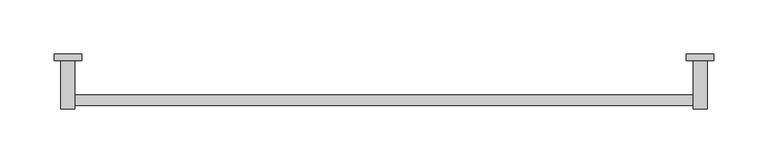
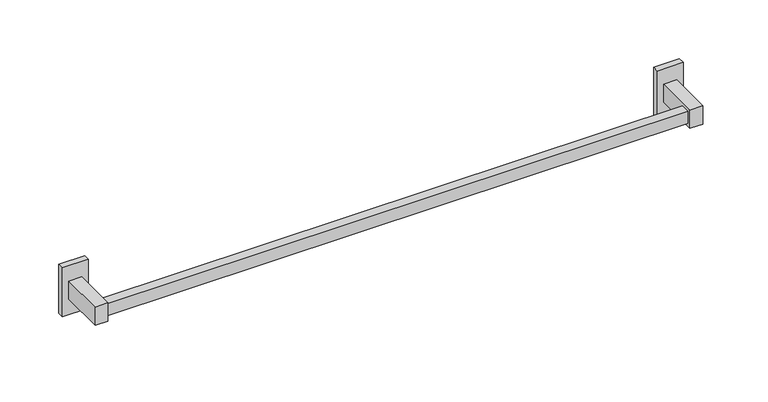
"""IFC4 building model written with IfcOpenShell, lengths in millimetres: proxy geometry, Towel Bar - NON-COLLECTUS : -."""

from ifc_helpers import new_model, si_unit, frame, origin, origin_with_axes, place, context, project, spatial, polyline, outline, extrude, source, transform, mapped, element, save


def specialty_equipment_6c124a1e(model_context):
    return source(origin(), model_context, "Body", "SweptSolid", [
        extrude(outline(polyline([(292.29939, -38.1), (292.29939, -47.625), (-292.29939, -47.625), (-292.29939, -38.1), (292.29939, -38.1)])), frame((0.0, 0.0, 19.05), z_axis=(0.0, 0.0, 1.0), x_axis=(1.0, 0.0, 0.0)), (0.0, 0.0, 1.0), 12.7),
        extrude(outline(polyline([(-298.64939, -6.35), (-285.94939, -6.35), (-285.94939, -50.8), (-298.64939, -50.8), (-298.64939, -6.35)])), frame((0.0, 0.0, 15.875), z_axis=(0.0, 0.0, 1.0), x_axis=(1.0, 0.0, 0.0)), (0.0, 0.0, 1.0), 19.05),
        extrude(outline(polyline([(285.94939, -6.35), (298.64939, -6.35), (298.64939, -50.8), (285.94939, -50.8), (285.94939, -6.35)])), frame((0.0, 0.0, 15.875), z_axis=(0.0, 0.0, 1.0), x_axis=(1.0, 0.0, 0.0)), (0.0, 0.0, 1.0), 19.05),
        extrude(outline(polyline([(-304.99939, 0.0), (-279.59939, 0.0), (-279.59939, -6.35), (-304.99939, -6.35), (-304.99939, 0.0)])), origin_with_axes(), (0.0, 0.0, 1.0), 50.8),
        extrude(outline(polyline([(279.59939, 0.0), (304.99939, 0.0), (304.99939, -6.35), (279.59939, -6.35), (279.59939, 0.0)])), origin_with_axes(), (0.0, 0.0, 1.0), 50.8),
    ])


if __name__ == "__main__":
    model = new_model("IFC4")
    model_context = context("Model", 3, world=origin())
    ifc_project = project(units=[si_unit("LENGTHUNIT", "METRE", prefix="MILLI")], contexts=[model_context])
    site = spatial("IfcSite", under=ifc_project)
    building = spatial("IfcBuilding", under=site)
    placement = place(None, origin())
    specialty_equipment_shape = specialty_equipment_6c124a1e(model_context)
    element("IfcBuildingElementProxy", 1, Name="Towel Bar - NON-COLLECTUS : -", ObjectType="Towel Bar - NON-COLLECTUS : -", at=placement, inside=building, context=model_context, shape_type="MappedRepresentation", body=[
        mapped(specialty_equipment_shape, transform((0.0, 0.0, 0.0), x_axis=(1.0, 0.0, 0.0), y_axis=(0.0, 1.0, 0.0), z_axis=(0.0, 0.0, 1.0))),
    ])
    save(model, "model.ifc")

# Revit data of these elements
# Type "Towel Bar - NON-COLLECTUS : -"
#   External ID [instance default] = ""
#   Width [instance default] = 609.6 mm
#   Height = 50.8 mm
#   Depth = 50.8 mm
#   Material = Light Grey
#   Default Elevation = 0
# Element 1 (IfcBuildingElementProxy, "Towel Bar - NON-COLLECTUS : -")
#   Width = 609.999 mm
#   Materials on its faces: "Light Grey"
# Materials
#   "Light Grey": class "Generic", colour RGB 215 215 215, transparency 0, Cost = 0
